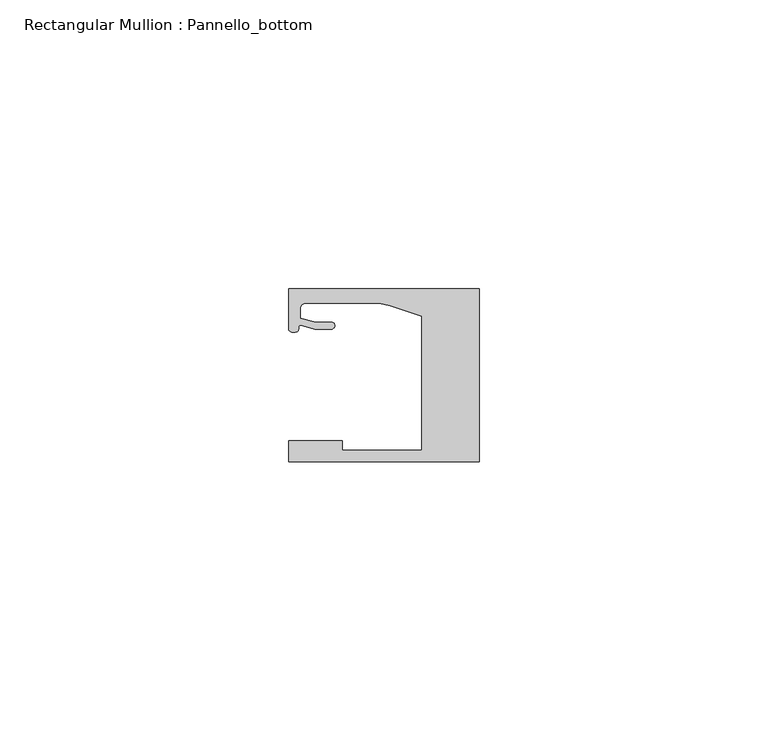
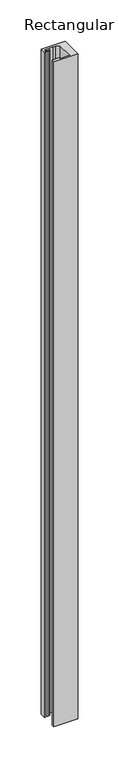
"""IFC4 building model written with IfcOpenShell, lengths in millimetres: member geometry, Rectangular Mullion : Pannello_bottom."""

from ifc_helpers import new_model, si_unit, frame, origin, place, context, project, spatial, polyline, circle_curve, source, transform, mapped, element, save
from ifc_brep_helpers import plane_surface, cylinder_surface, revolved_surface, extruded_surface, spline_curve, advanced_brep


def rectangular_mullion_pannello_bottom_9a96a0aa(model_context):
    return source(origin(), model_context, "Body", "AdvancedBrep", [
        advanced_brep(
        [(-33.0, -15.0, 0.0), (0.0, -15.0, 0.0), (0.0, 15.0, 0.0), (-33.0000135, 15.0, 0.0), (-33.0000135, 8.0000472, 0.0), (-30.9223017, 8.6490241, 0.0), (-28.4999305, 7.9999523, 0.0), (-25.59998, 7.9999523, 0.0), (-25.59998, 9.1999523, 0.0), (-28.3419477, 9.1999523, 0.0), (-31.0, 9.9121746, 0.0), (-31.0, 11.4999419, 0.0), (-30.0000002, 12.4999419, 0.0), (-18.5493024, 12.4999438, 0.0), (-15.4591336, 12.0105099, 0.0), (-9.9999723, 10.2367227, 0.0), (-9.9999723, -13.0000004, 0.0), (-23.700041, -13.0000004, 0.0), (-23.700041, -11.3000004, 0.0), (-33.0, -11.3000004, 0.0), (-33.0, -15.0, -980.0), (-33.0, -11.3000004, -980.0), (-23.700041, -11.3000004, -980.0), (-23.700041, -13.0000004, -980.0), (-9.9999723, -13.0000004, -980.0), (-9.9999723, 10.2367227, -980.0), (-15.4591336, 12.0105099, -980.0), (-18.5493024, 12.4999438, -980.0), (-30.0000002, 12.4999419, -980.0), (-31.0, 11.4999419, -980.0), (-31.0, 9.9121746, -980.0), (-28.3419477, 9.1999523, -980.0), (-25.59998, 9.1999523, -980.0), (-25.59998, 7.9999523, -980.0), (-28.4999305, 7.9999523, -980.0), (-30.9223017, 8.6490241, -980.0), (-33.0000135, 8.0000472, -980.0), (-33.0000135, 15.0, -980.0), (0.0, 15.0, -980.0), (0.0, -15.0, -980.0)],
        [
            (0, 1),
            (1, 2),
            (2, 3),
            (3, 4),
            (4, 5, spline_curve(3, [(-33.0000135, 8.0000472, 0.0), (-33.0000135, 7.457047519, 0.0), (-32.262327879, 7.456527435, 0.0), (-31.357433266, 7.563996614, 0.0), (-31.305645054, 7.690065204, 0.0), (-31.298563602, 8.366228555, 0.0), (-31.312054066, 8.717747958, 0.0), (-30.9223017, 8.6490241, 0.0)], [4, 2, 2, 4], [0.0, 0.0027053965905959043, 0.0058611956533709, 0.007702013405570312])),
            (5, 6),
            (6, 7),
            (7, 8, circle_curve(frame((-25.59998, 8.5999523, 0.0), z_axis=(0.0, 0.0, 1.0), x_axis=(0.0, 1.0, 0.0)), 0.6)),
            (8, 9),
            (9, 10),
            (10, 11),
            (11, 12, circle_curve(frame((-30.0, 11.4999419, 0.0), z_axis=(0.0, 0.0, -1.0), x_axis=(0.0, 1.0, 0.0)), 1.0)),
            (12, 13),
            (13, 14, circle_curve(frame((-18.5493007, 2.4999438, 0.0), z_axis=(0.0, 0.0, -1.0), x_axis=(0.0, 1.0, 0.0)), 10.0)),
            (14, 15),
            (15, 16),
            (16, 17),
            (17, 18),
            (18, 19),
            (19, 0),
            (20, 21),
            (21, 22),
            (22, 23),
            (23, 24),
            (24, 25),
            (25, 26),
            (26, 27, circle_curve(frame((-18.5493007, 2.4999438, -980.0), z_axis=(0.0, 0.0, 1.0), x_axis=(0.0, 1.0, 0.0)), 10.0)),
            (27, 28),
            (28, 29, circle_curve(frame((-30.0, 11.4999419, -980.0), z_axis=(0.0, 0.0, 1.0), x_axis=(0.0, 1.0, 0.0)), 1.0)),
            (29, 30),
            (30, 31),
            (31, 32),
            (32, 33, circle_curve(frame((-25.59998, 8.5999523, -980.0), z_axis=(0.0, 0.0, -1.0), x_axis=(0.0, 1.0, 0.0)), 0.6)),
            (33, 34),
            (34, 35),
            (35, 36, spline_curve(3, [(-30.9223017, 8.6490241, -980.0), (-31.312054066, 8.717747958, -980.0), (-31.298563602, 8.366228555, -980.0), (-31.305645054, 7.690065204, -980.0), (-31.357433266, 7.563996614, -980.0), (-32.262327879, 7.456527435, -980.0), (-33.0000135, 7.457047519, -980.0), (-33.0000135, 8.0000472, -980.0)], [4, 2, 2, 4], [0.0, 0.001840817752199412, 0.004996616814974408, 0.007702013405570312])),
            (36, 37),
            (37, 38),
            (38, 39),
            (39, 20),
            (0, 20),
            (39, 1),
            (38, 2),
            (37, 3),
            (36, 4),
            (35, 5),
            (34, 6),
            (33, 7),
            (32, 8),
            (31, 9),
            (30, 10),
            (29, 11),
            (28, 12),
            (27, 13),
            (26, 14),
            (25, 15),
            (24, 16),
            (23, 17),
            (22, 18),
            (21, 19),
        ],
        [
            plane_surface(frame((0.0, -36.2491502, 0.0), z_axis=(0.0, 0.0, 1.0), x_axis=(-1.0, 0.0, 0.0))),
            plane_surface(frame((0.0, -36.2491502, -980.0), z_axis=(0.0, 0.0, -1.0), x_axis=(-1.0, 0.0, 0.0))),
            plane_surface(frame((-33.0, -15.0, 0.0), z_axis=(0.0, -1.0, 0.0), x_axis=(0.0, 0.0, -1.0))),
            plane_surface(frame((0.0, -15.0, 0.0), z_axis=(1.0, 0.0, 0.0), x_axis=(0.0, 0.0, -1.0))),
            plane_surface(frame((0.0, 15.0, 0.0), z_axis=(0.0, 1.0, 0.0), x_axis=(0.0, 0.0, -1.0))),
            plane_surface(frame((-33.0000135, 15.0, 0.0), z_axis=(-1.0, 0.0, 0.0), x_axis=(0.0, 0.0, -1.0))),
            extruded_surface(spline_curve(3, [(-33.0000135, 8.0000472, -980.0), (-33.0000135, 7.457047519, -980.0), (-32.262327879, 7.456527435, -980.0), (-31.357433266, 7.563996614, -980.0), (-31.305645054, 7.690065204, -980.0), (-31.298563602, 8.366228555, -980.0), (-31.312054066, 8.717747958, -980.0), (-30.9223017, 8.6490241, -980.0)], [4, 2, 2, 4], [0.0, 0.0027053965905959043, 0.0058611956533709, 0.007702013405570312]), (0.0, 0.0, 980.0), 980.0),
            plane_surface(frame((-30.9223017, 8.6490241, 0.0), z_axis=(-0.25881883200192934, -0.9659258833891746, 0.0), x_axis=(0.0, 0.0, -1.0))),
            plane_surface(frame((-28.4999305, 7.9999523, 0.0), z_axis=(0.0, -1.0, 0.0), x_axis=(0.0, 0.0, -1.0))),
            cylinder_surface(frame((-25.59998, 8.5999523, 0.0), z_axis=(0.0, 0.0, 1.0), x_axis=(0.0, 1.0, 0.0)), 0.6),
            plane_surface(frame((-25.59998, 9.1999523, 0.0), z_axis=(0.0, 1.0, 0.0), x_axis=(0.0, 0.0, -1.0))),
            plane_surface(frame((-28.3419477, 9.1999523, 0.0), z_axis=(0.25881883204288636, 0.9659258833782002, 0.0), x_axis=(0.0, 0.0, -1.0))),
            plane_surface(frame((-31.0, 9.9121746, 0.0), z_axis=(1.0, 0.0, 0.0), x_axis=(0.0, 0.0, -1.0))),
            revolved_surface(polyline([(-30.0, 12.4999419, -980.0), (-30.0, 12.4999419, 0.0)]), (-30.0, 11.4999419, 0.0), (0.0, 0.0, -1.0)),
            plane_surface(frame((-30.0000002, 12.4999419, 0.0), z_axis=(1.6923026533778639e-07, -0.9999999999999858, 0.0), x_axis=(0.0, 0.0, -1.0))),
            revolved_surface(polyline([(-18.5493007, 12.4999438, -980.0), (-18.5493007, 12.4999438, 0.0)]), (-18.5493007, 2.4999438, 0.0), (0.0, 0.0, -1.0)),
            plane_surface(frame((-15.4591336, 12.0105099, 0.0), z_axis=(-0.30901670911956314, -0.9510566089801992, 0.0), x_axis=(0.0, 0.0, -1.0))),
            plane_surface(frame((-9.9999723, 10.2367227, 0.0), z_axis=(-1.0, 0.0, 0.0), x_axis=(0.0, 0.0, -1.0))),
            plane_surface(frame((-9.9999723, -13.0000004, 0.0), z_axis=(0.0, 1.0, 0.0), x_axis=(0.0, 0.0, -1.0))),
            plane_surface(frame((-23.700041, -13.0000004, 0.0), z_axis=(1.0, 0.0, 0.0), x_axis=(0.0, 0.0, -1.0))),
            plane_surface(frame((-23.700041, -11.3000004, 0.0), z_axis=(0.0, 1.0, 0.0), x_axis=(0.0, 0.0, -1.0))),
            plane_surface(frame((-33.0, -11.3000004, 0.0), z_axis=(-1.0, 0.0, 0.0), x_axis=(0.0, 0.0, -1.0))),
        ],
        [
            (0, [[1, 2, 3, 4, 5, 6, 7, 8, 9, 10, 11, 12, 13, 14, 15, 16, 17, 18, 19, 20]]),
            (1, [[21, 22, 23, 24, 25, 26, 27, 28, 29, 30, 31, 32, 33, 34, 35, 36, 37, 38, 39, 40]]),
            (2, [[-1, 41, -40, 42]]),
            (3, [[-2, -42, -39, 43]]),
            (4, [[-3, -43, -38, 44]]),
            (5, [[-4, -44, -37, 45]]),
            (6, [[-5, -45, -36, 46]]),
            (7, [[-6, -46, -35, 47]]),
            (8, [[-7, -47, -34, 48]]),
            (9, [[-8, -48, -33, 49]]),
            (10, [[-9, -49, -32, 50]]),
            (11, [[-10, -50, -31, 51]]),
            (12, [[-11, -51, -30, 52]]),
            (13, [[-12, -52, -29, 53]]),
            (14, [[-13, -53, -28, 54]]),
            (15, [[-14, -54, -27, 55]]),
            (16, [[-15, -55, -26, 56]]),
            (17, [[-16, -56, -25, 57]]),
            (18, [[-17, -57, -24, 58]]),
            (19, [[-18, -58, -23, 59]]),
            (20, [[-19, -59, -22, 60]]),
            (21, [[-20, -60, -21, -41]]),
        ],
    ),
    ])


if __name__ == "__main__":
    model = new_model("IFC4")
    model_context = context("Model", 3, world=origin())
    ifc_project = project(units=[si_unit("LENGTHUNIT", "METRE", prefix="MILLI")], contexts=[model_context])
    site = spatial("IfcSite", under=ifc_project)
    building = spatial("IfcBuilding", under=site)
    placement = place(None, origin())
    rectangular_mullion_pannello_bottom_shape = rectangular_mullion_pannello_bottom_9a96a0aa(model_context)
    element("IfcMember", 1, ObjectType="Rectangular Mullion : Pannello_bottom", at=placement, inside=building, context=model_context, shape_type="MappedRepresentation", body=[
        mapped(rectangular_mullion_pannello_bottom_shape, transform((0.0, 0.0, 0.0), x_axis=(1.0, 0.0, 0.0), y_axis=(0.0, 1.0, 0.0), z_axis=(0.0, 0.0, 1.0))),
    ])
    save(model, "model.ifc")

# Revit data of these elements
# Type "Rectangular Mullion : Pannello_bottom"
#   built-in parameter 1007322 = 0.0984252 (stored number, unit not read)
#   built-in parameter 1007321 = 0.0328083 (stored number, unit not read)
#   built-in parameter 1007320 = 0 (stored number, unit not read)
